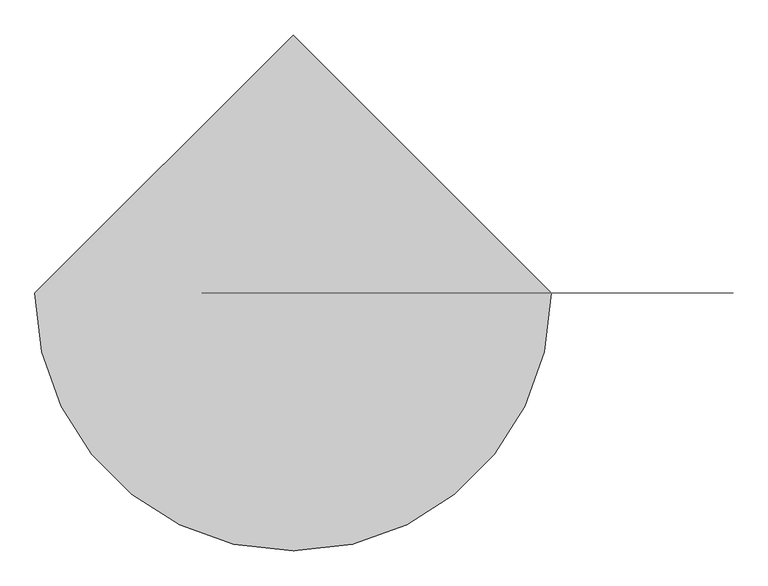
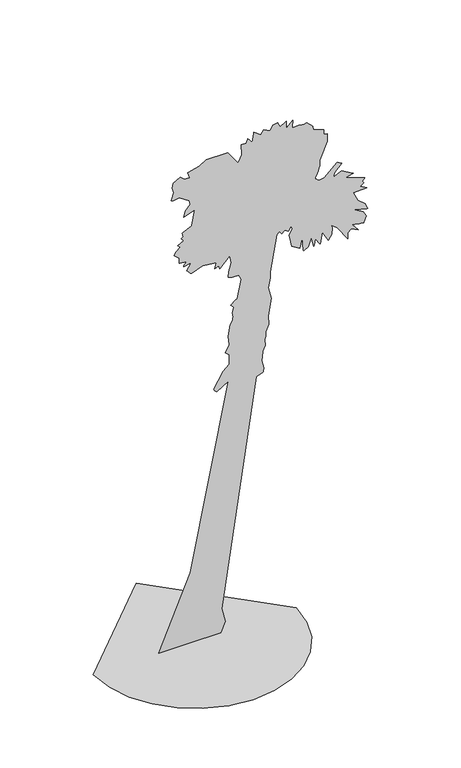
"""IFC4 building model written with IfcOpenShell, lengths in millimetres: proxy geometry, california fan palm 26448 : california fan palm 26448."""

import ifcopenshell
import ifcopenshell.guid

model = None  # the IFC model being written
_history = None  # IfcOwnerHistory: only IFC2X3 demands one
_inside = {}  # id of a spatial element -> (the spatial element, [elements in it])
_under = {}  # id of a project, library or spatial element -> (it, [spatial elements below it])
_declared = {}  # id of a project -> (the project, [libraries it declares])
_typed = {}  # id of a type object -> (the type object, [elements of that type])
_made_of = {}  # id of a material, layer set ... -> (it, [elements and type objects made of it])


def new_model(schema):
    """Start an empty IFC model of exactly this schema.

    Asked for "IFC4X3", IfcOpenShell would pick the latest addendum, in which some entities
    have other attributes; the version numbers below select the first issue.
    IFC2X3 requires an IfcOwnerHistory on every rooted entity: one is made here for all.
    """
    global model, _history
    if schema == "IFC4X3":
        model = ifcopenshell.file(schema_version=(4, 3, 0, 0))
    else:
        model = ifcopenshell.file(schema=schema)
    _inside.clear()
    _under.clear()
    _declared.clear()
    _typed.clear()
    _made_of.clear()
    _history = None
    if model.schema == "IFC2X3":
        org = make("IfcOrganization", Name="unknown")
        user = make(
            "IfcPersonAndOrganization",
            ThePerson=make("IfcPerson", FamilyName="unknown"),
            TheOrganization=org,
        )
        app = make(
            "IfcApplication",
            ApplicationDeveloper=org,
            Version="unknown",
            ApplicationFullName="unknown",
            ApplicationIdentifier="unknown",
        )
        _history = make(
            "IfcOwnerHistory",
            OwningUser=user,
            OwningApplication=app,
            ChangeAction="ADDED",
            CreationDate=0,
        )
    return model


def make(cls, **values):
    """One entity of the class cls with the attributes given. An attribute that is None is left unset."""
    return model.create_entity(
        cls, **{name: value for name, value in values.items() if value is not None}
    )


def rooted(cls, **values):
    """An entity with a GlobalId (a new one), such as an element, a storey or a relation."""
    return make(cls, GlobalId=ifcopenshell.guid.new(), OwnerHistory=_history, **values)


def si_unit(unit_type, name, prefix=None):
    """IfcSIUnit, for example si_unit("LENGTHUNIT", "METRE", prefix="MILLI")."""
    return make("IfcSIUnit", UnitType=unit_type, Prefix=prefix, Name=name)


def assignment(units):
    """IfcUnitAssignment: the units of a project."""
    return None if units is None else make("IfcUnitAssignment", Units=units)


def point(xyz):
    """IfcCartesianPoint."""
    return None if xyz is None else make("IfcCartesianPoint", Coordinates=xyz)


def direction(xyz):
    """IfcDirection."""
    return None if xyz is None else make("IfcDirection", DirectionRatios=xyz)


def frame(location, z_axis=None, x_axis=None):
    """IfcAxis2Placement3D, a coordinate frame: its origin and axes. An axis left out is left unset."""
    return make(
        "IfcAxis2Placement3D",
        Location=point(location),
        Axis=direction(z_axis),
        RefDirection=direction(x_axis),
    )


def origin():
    """The frame at (0, 0, 0) with its axes left unset."""
    return frame((0.0, 0.0, 0.0))


def place(relative_to, where):
    """IfcLocalPlacement: puts the frame where relative to a parent placement (None: the world)."""
    return make(
        "IfcLocalPlacement", PlacementRelTo=relative_to, RelativePlacement=where
    )


def context(
    kind, dimensions, precision=None, world=None, true_north=None, identifier=None
):
    """IfcGeometricRepresentationContext, for example the 3D "Model" context."""
    return make(
        "IfcGeometricRepresentationContext",
        ContextIdentifier=identifier,
        ContextType=kind,
        CoordinateSpaceDimension=dimensions,
        Precision=precision,
        WorldCoordinateSystem=world,
        TrueNorth=true_north,
    )


def project(units=None, contexts=None):
    """IfcProject with its units and contexts."""
    return rooted(
        "IfcProject",
        Name="project",
        RepresentationContexts=contexts,
        UnitsInContext=assignment(units),
    )


def spatial(cls, under=None, at=None, **own):
    """A site, building, storey or space (cls), placed at a placement, below another one or the project."""
    s = rooted(cls, ObjectPlacement=at, **own)
    if under is not None:
        _under.setdefault(under.id(), (under, []))[1].append(s)
    return s


def point_list(points):
    """IfcCartesianPointList2D or 3D."""
    cls = (
        "IfcCartesianPointList2D" if len(points[0]) == 2 else "IfcCartesianPointList3D"
    )
    return make(cls, CoordList=points)


def triangles(points, corners, closed=None, point_numbers=None):
    """IfcTriangulatedFaceSet: each triangle names its three corners, points numbered from 1."""
    return make(
        "IfcTriangulatedFaceSet",
        Coordinates=point_list(points),
        Closed=closed,
        CoordIndex=corners,
        PnIndex=point_numbers,
    )


def shape(context_of_items, identifier, shape_type, items):
    """IfcShapeRepresentation: the items that make up one representation, for example the "Body"."""
    return make(
        "IfcShapeRepresentation",
        ContextOfItems=context_of_items,
        RepresentationIdentifier=identifier,
        RepresentationType=shape_type,
        Items=items,
    )


def source(mapping_origin, context_of_items, identifier, shape_type, items):
    """IfcRepresentationMap: a shape defined once, which mapped items show again and again."""
    return make(
        "IfcRepresentationMap",
        MappingOrigin=mapping_origin,
        MappedRepresentation=shape(context_of_items, identifier, shape_type, items),
    )


def transform(
    local_origin,
    x_axis=None,
    y_axis=None,
    z_axis=None,
    scale=None,
    scale2=None,
    scale3=None,
    uniform=True,
):
    """IfcCartesianTransformationOperator3D, or its non-uniform kind. x_axis, y_axis, z_axis: its Axis1, 2, 3."""
    if uniform:
        return make(
            "IfcCartesianTransformationOperator3D",
            Axis1=direction(x_axis),
            Axis2=direction(y_axis),
            LocalOrigin=point(local_origin),
            Scale=scale,
            Axis3=direction(z_axis),
        )
    return make(
        "IfcCartesianTransformationOperator3DnonUniform",
        Axis1=direction(x_axis),
        Axis2=direction(y_axis),
        LocalOrigin=point(local_origin),
        Scale=scale,
        Axis3=direction(z_axis),
        Scale2=scale2,
        Scale3=scale3,
    )


def mapped(mapping_source, mapping_target):
    """IfcMappedItem: shows the shape of a source again, moved by a transform."""
    return make(
        "IfcMappedItem", MappingSource=mapping_source, MappingTarget=mapping_target
    )


def made_of(thing, what):
    """Note that an element or type object is made of a material, layer set ...; save() writes the relation."""
    if what is not None:
        _made_of.setdefault(what.id(), (what, []))[1].append(thing)
    return thing


def element(
    cls,
    number,
    at=None,
    inside=None,
    cuts=None,
    type_object=None,
    material=None,
    context=None,
    identifier="Body",
    shape_type=None,
    held_by="IfcProductDefinitionShape",
    body=None,
    shapes=None,
    **own,
):
    """One element of the class cls, such as IfcWall. Its Tag is "e" and its number.

    at: its placement. inside: the storey or other place that contains it. cuts: it is an
    opening in that element (IfcRelVoidsElement). A single representation is given by context,
    identifier, shape_type and body (its items); several are given by shapes. held_by: the class
    of the entity that holds the representations. save() writes the other relations.
    """
    e = rooted(cls, Tag="e%d" % number, ObjectPlacement=at, **own)
    if body is not None:
        shapes = [shape(context, identifier, shape_type, body)]
    if shapes is not None:
        e.Representation = make(held_by, Representations=shapes)
    if inside is not None:
        _inside.setdefault(inside.id(), (inside, []))[1].append(e)
    if cuts is not None:
        rooted(
            "IfcRelVoidsElement", RelatingBuildingElement=cuts, RelatedOpeningElement=e
        )
    if type_object is not None:
        _typed.setdefault(type_object.id(), (type_object, []))[1].append(e)
    return made_of(e, material)


def aggregate(whole, parts):
    """IfcRelAggregates: a whole, such as a stair, and the parts it consists of."""
    return rooted("IfcRelAggregates", RelatingObject=whole, RelatedObjects=parts)


def save(model, path):
    """Write the relations noted so far, then the file.

    IfcRelAggregates (storeys below a building ...), IfcRelContainedInSpatialStructure (elements
    in a storey), IfcRelDefinesByType, IfcRelAssociatesMaterial and IfcRelDeclares: one each for
    every whole, place, type object, material and project.
    """
    for whole, parts in _under.values():
        aggregate(whole, parts)
    for where, things in _inside.values():
        rooted(
            "IfcRelContainedInSpatialStructure",
            RelatedElements=things,
            RelatingStructure=where,
        )
    for kind, things in _typed.values():
        rooted("IfcRelDefinesByType", RelatedObjects=things, RelatingType=kind)
    for what, things in _made_of.values():
        rooted("IfcRelAssociatesMaterial", RelatedObjects=things, RelatingMaterial=what)
    for by, libraries in _declared.values():
        rooted("IfcRelDeclares", RelatingContext=by, RelatedDefinitions=libraries)
    model.write(path)


def entourage_5d10e8ee(model_context):
    return source(origin(), model_context, "Body", "Tessellation", [
        triangles([(-2230.6788128, 0.0, 0.0), (-2171.7626415, -511.0878808, 0.0), (-2003.8055969, -980.4489481, 0.0), (-1740.3231331, -1394.6991714, 0.0), (-1394.6991714, -1740.3231331, 0.0), (-980.4489481, -2003.8055969, 0.0), (-511.0878808, -2171.7626415, 0.0), (0.0, -2230.6788128, 0.0), (511.0878808, -2171.7626415, 0.0), (980.4489481, -2003.8055969, 0.0), (1394.6991714, -1740.3231331, 0.0), (1740.3231331, -1394.6991714, 0.0), (2003.8055969, -980.4489481, 0.0), (2171.7626415, -511.0878808, 0.0), (2230.6788128, 0.0, 0.0), (0.0, 2230.6788128, 0.0), (1664.2176041, 0.0, 11296.8139435), (1716.9665646, 0.0, 11409.2663818), (1822.5957275, 0.0, 11429.86745), (1831.5184387, 0.0, 11420.4191895), (1867.2094288, 0.0, 11334.210498), (1869.9649292, 0.0, 11312.4281067), (2015.4839539, 0.0, 11398.3751862), (2017.4521477, 0.0, 11231.8609314), (2029.3928432, 0.0, 11239.7348694), (2152.211364, 0.0, 11376.1997955), (2149.9806862, 0.0, 11207.8484436), (2152.473848, 0.0, 11197.3514099), (2288.0203709, 0.0, 11209.0297668), (2303.3726315, 0.0, 11206.5368958), (2322.5303284, 0.0, 11201.6813782), (2343.1312511, 0.0, 11196.0398621), (2362.6825287, 0.0, 11190.7901825), (2378.8220959, 0.0, 11187.6415375), (2392.5998886, 0.0, 11190.1344086), (2470.1486435, 0.0, 11209.9483154), (2596.1165359, 0.0, 11074.5333252), (2606.0888924, 0.0, 10999.6088287), (2622.0972176, 0.0, 10989.2420197), (2841.8846741, 0.0, 10912.2188141), (2834.4054794, 0.0, 10804.8835052), (2918.2526871, 0.0, 10792.4179871), (2914.3162994, 0.0, 10622.229538), (2746.3591095, 0.0, 10233.4358276), (2746.8840775, 0.0, 10223.5945679), (2748.4586906, 0.0, 10207.4548553), (2750.2957878, 0.0, 10187.6409485), (2752.0014977, 0.0, 10166.9096558), (2753.1825302, 0.0, 10147.8829102), (2752.5264656, 0.0, 10129.2503265), (2746.4904968, 0.0, 10101.3008698), (2732.5814621, 0.0, 10059.0487976), (2713.4239105, 0.0, 10006.1694672), (2692.2981651, 0.0, 9950.4019409), (2672.3531616, 0.0, 9899.7527069), (2657.000901, 0.0, 9861.830603), (2649.652803, 0.0, 9844.3793427), (2655.1638039, 0.0, 9835.7194061), (2666.9732574, 0.0, 9823.9096619), (2682.588002, 0.0, 9810.3942078), (2699.9087471, 0.0, 9796.4857544), (2716.8356209, 0.0, 9783.8888489), (2731.1382362, 0.0, 9773.7848145), (2743.9973351, 0.0, 9768.1421356), (2762.8924026, 0.0, 9771.5535553), (2783.4934708, 0.0, 9776.0149109), (2805.8002487, 0.0, 9781.0018158), (2826.6638008, 0.0, 9785.987558), (2846.6085136, 0.0, 9790.8430756), (3136.3344337, 0.0, 10050.2574738), (3236.3213539, 0.0, 9997.9025299), (3081.0921661, 0.0, 9835.4566315), (3047.3698059, 0.0, 9739.0125183), (3230.9414497, 0.0, 9821.1540161), (3471.198587, 0.0, 9683.1141861), (3486.2886543, 0.0, 9668.9429581), (3314.6575607, 0.0, 9631.5464035), (3745.0472786, 0.0, 9483.4031204), (3683.7693329, 0.0, 9424.0927872), (3714.4738541, 0.0, 9372.0000366), (3638.7619057, 0.0, 9318.7265442), (3786.6429955, 0.0, 9226.0874313), (3491.0122032, 0.0, 9221.3638824), (3589.5558975, 0.0, 9011.2860077), (3750.2957954, 0.0, 8872.4595978), (3802.1263527, 0.0, 8753.0523514), (3802.3888367, 0.0, 8743.6046722), (3785.8555435, 0.0, 8741.1118011), (3521.0609505, 0.0, 8817.3484268), (3708.9628532, 0.0, 8702.927504), (3773.3900253, 0.0, 8589.950679), (3773.3900253, 0.0, 8579.0594833), (3723.3965652, 0.0, 8451.5172684), (3722.7405006, 0.0, 8439.9702988), (3582.3388962, 0.0, 8467.3942062), (3469.6239738, 0.0, 8483.9274994), (3593.2298012, 0.0, 8317.5452133), (3446.0050667, 0.0, 8391.1575806), (3364.6510208, 0.0, 8326.0743439), (3364.9135048, 0.0, 8189.871611), (3139.2211761, 0.0, 8528.6724426), (3001.4438301, 0.0, 8636.6635254), (3024.9316406, 0.0, 8566.4625778), (3019.5517365, 0.0, 8420.4185852), (2940.4283684, 0.0, 8304.6861145), (2805.2752808, 0.0, 8540.6129929), (2760.1370476, 0.0, 8283.0351105), (2749.7708199, 0.0, 8292.6141769), (2653.9827713, 0.0, 8439.0517502), (2626.9524445, 0.0, 8297.7313065), (2620.9164757, 0.0, 8283.0351105), (2579.5832428, 0.0, 8449.8115585), (2567.9048859, 0.0, 8491.0131134), (2498.0978096, 0.0, 8313.2152451), (2400.9976318, 0.0, 8247.8692337), (2391.943824, 0.0, 8267.9453339), (2363.6010773, 0.0, 8580.3716125), (2316.2318756, 0.0, 8342.0826691), (2134.3659416, 0.0, 8446.7931381), (2079.2550613, 0.0, 8724.578508), (2142.2390076, 0.0, 8848.577916), (2140.5331524, 0.0, 8863.4054993), (2136.7278614, 0.0, 8876.1332108), (2131.7416832, 0.0, 8889.1236969), (2126.493021, 0.0, 8901.1956345), (2118.2263744, 0.0, 8911.5618622), (2064.821204, 0.0, 8836.1123978), (2061.278397, 0.0, 8825.74617), (1984.5168034, 0.0, 8874.5588882), (1971.6575592, 0.0, 8870.8846939), (1961.5539608, 0.0, 8863.4054993), (1929.4059231, 0.0, 8825.3525894), (1918.6462601, 0.0, 8820.3662659), (1866.2908802, 0.0, 8885.1873093), (1856.7121044, 0.0, 8882.4316635), (1845.5587154, 0.0, 8875.3460495), (1833.7492619, 0.0, 8865.5047897), (1822.2021469, 0.0, 8854.2200134), (1811.8360645, 0.0, 8842.9358185), (1800.8139175, 0.0, 8829.6825577), (1660.4123131, 0.0, 8018.3716141), (1661.7244423, 0.0, 7883.0874298), (1618.029435, 0.0, 7666.7116837), (1684.0312202, 0.0, 7392.9946701), (1613.6993214, 0.0, 6996.1962158), (1630.1013725, 0.0, 6826.0083481), (1628.2642754, 0.0, 6813.1492493), (1565.0179905, 0.0, 6658.9697067), (1565.0179905, 0.0, 6648.2098984), (1564.7555065, 0.0, 6634.432251), (1564.2306839, 0.0, 6619.0802811), (1564.0994419, 0.0, 6603.3341492), (1564.3619259, 0.0, 6588.6379532), (1566.3301197, 0.0, 6572.10466), (1566.0677811, 0.0, 6561.3448517), (1562.0000061, 0.0, 6547.1736237), (1555.9640373, 0.0, 6528.54104), (1549.2720039, 0.0, 6508.2021652), (1542.9736965, 0.0, 6489.176001), (1536.6752438, 0.0, 6470.41203), (1549.6657299, 0.0, 6358.8781403), (1547.8286327, 0.0, 6349.0368805), (1519.879612, 0.0, 6273.9809967), (1509.1198036, 0.0, 6246.9500885), (1500.7219151, 0.0, 6225.4310532), (1496.3918015, 0.0, 6213.6213089), (1479.0712017, 0.0, 6016.271727), (1517.6489342, 0.0, 5834.537471), (1516.3366596, 0.0, 5819.7098877), (1513.5811592, 0.0, 5801.6016907), (1510.1695942, 0.0, 5782.7069138), (1506.6266418, 0.0, 5765.255072), (1502.4277702, 0.0, 5747.9346176), (1492.9802364, 0.0, 5740.5862289), (1349.2983089, 0.0, 5680.8828964), (595.4600201, 0.0, 547.8284798), (673.9273962, 0.0, 229.1038392), (568.9542978, 0.0, 0.0), (-790.1851255, 0.0, 0.0), (-95.6567521, 0.0, 1632.0695663), (739.9292542, 0.0, 5779.1641068), (737.436165, 0.0, 5791.104657), (723.0023804, 0.0, 5788.3490112), (497.4413664, 0.0, 5642.1742126), (481.6954162, 0.0, 5644.929277), (467.1303895, 0.0, 5652.2776657), (442.9865507, 0.0, 5676.2901535), (421.4670794, 0.0, 5718.8044189), (623.2778715, 0.0, 6073.2199951), (759.0868784, 0.0, 6187.6403366), (764.0731293, 0.0, 6248.393605), (761.5799675, 0.0, 6329.354361), (759.4805317, 0.0, 6365.176593), (758.0371605, 0.0, 6391.1569839), (755.0191761, 0.0, 6405.9845673), (666.1856449, 0.0, 6482.8775482), (763.548234, 0.0, 6634.301445), (735.9927938, 0.0, 6838.6052536), (766.6974604, 0.0, 7041.3347397), (776.8010588, 0.0, 7092.5089417), (840.0474163, 0.0, 7190.1337967), (839.522521, 0.0, 7202.4679276), (839.653763, 0.0, 7214.1462845), (840.3098276, 0.0, 7226.8745773), (841.2283762, 0.0, 7239.2087082), (843.0654007, 0.0, 7253.5113235), (843.459054, 0.0, 7264.4025192), (841.4907875, 0.0, 7278.1801666), (838.3415611, 0.0, 7296.025589), (834.5362701, 0.0, 7315.1831406), (830.9934631, 0.0, 7332.8971756), (827.1881721, 0.0, 7349.5618561), (858.9425566, 0.0, 7476.4482971), (792.0222227, 0.0, 7542.3186951), (801.9946518, 0.0, 7559.2455688), (893.5836834, 0.0, 7626.0345154), (936.6226988, 0.0, 7645.4548416), (1020.8635597, 0.0, 8067.9714935), (970.6076883, 0.0, 8186.4601913), (830.0749146, 0.0, 8178.4560287), (740.9790447, 0.0, 8214.1468735), (747.8022474, 0.0, 8345.4940887), (801.8634098, 0.0, 8532.8710236), (775.3576876, 0.0, 8707.5202469), (545.597802, 0.0, 8480.6468857), (527.0962787, 0.0, 8557.4084793), (442.0680385, 0.0, 8522.5053772), (472.772705, 0.0, 8646.6361725), (175.6987596, 0.0, 8679.0464035), (149.3242611, 0.0, 8677.3406937), (-68.4949607, 0.0, 8593.099324), (-83.7160656, 0.0, 8594.6742279), (-100.2493315, 0.0, 8606.0898102), (-163.6268583, 0.0, 8679.0464035), (-174.6490235, 0.0, 8687.0505661), (-73.2187503, 0.0, 8837.8181076), (-247.211691, 0.0, 8810.3942001), (-243.8000715, 0.0, 8822.3347504), (-191.1822985, 0.0, 8889.9108582), (-182.5220168, 0.0, 8896.9970535), (-226.4795081, 0.0, 8901.4584091), (-326.8600634, 0.0, 8910.7747009), (-336.4388391, 0.0, 8914.1861206), (-338.5383113, 0.0, 9032.0184631), (-454.139976, 0.0, 9130.9554474), (-421.729527, 0.0, 9200.631427), (-316.4939446, 0.0, 9287.7592484), (-374.0979504, 0.0, 9343.1326126), (-245.112237, 0.0, 9404.9352356), (-247.8677738, 0.0, 9414.1207214), (-255.0846843, 0.0, 9424.7491425), (-300.8792001, 0.0, 9470.2812469), (-254.166172, 0.0, 9507.1528336), (-275.2920083, 0.0, 9598.0862366), (-268.468751, 0.0, 9606.3525925), (-79.1234862, 0.0, 9686.3947998), (-65.8706341, 0.0, 9707.3894485), (-0.1312164, 0.0, 10040.1546021), (-244.7185837, 0.0, 9956.7003937), (-207.9780029, 0.0, 10078.3383179), (-100.1181167, 0.0, 10203.780661), (-126.0989619, 0.0, 10300.0933868), (-346.8049579, 0.0, 10440.889444), (-468.442555, 0.0, 10419.7628265), (-522.8973707, 0.0, 10436.8210876), (-465.9494296, 0.0, 10603.5969543), (-492.9800108, 0.0, 10720.6421356), (-468.8362083, 0.0, 10823.2533142), (-318.9870701, 0.0, 10910.9061035), (-233.6964004, 0.0, 10839.2616394), (-108.1223157, 0.0, 10825.353186), (-151.5549389, 0.0, 10960.7681763), (96.9689176, 0.0, 11018.8971863), (255.6095432, 0.0, 11124.9197845), (725.2330582, 0.0, 11114.0285889), (954.2056372, 0.0, 10789.530954), (960.8976706, 0.0, 10798.7164398), (1037.2656109, 0.0, 10964.7051453), (1025.8498106, 0.0, 11198.2699585), (1137.9085957, 0.0, 11192.758667), (1136.4652245, 0.0, 11204.0440247), (1141.5826447, 0.0, 11231.8609314), (1162.0524708, 0.0, 11273.5886169), (1170.1878754, 0.0, 11283.6914886), (1265.188472, 0.0, 11172.5517609), (1295.1058319, 0.0, 11376.1997955), (1299.9609135, 0.0, 11390.6337982), (1447.8417126, 0.0, 11287.365683), (1520.9292572, 0.0, 11379.6112152)], [[15, 16, 1], [14, 15, 1], [14, 1, 2], [13, 14, 2], [13, 2, 3], [13, 3, 4], [12, 13, 4], [11, 12, 4], [11, 4, 5], [11, 5, 6], [11, 6, 7], [11, 7, 8], [11, 8, 9], [11, 9, 10], [266, 267, 268], [266, 268, 269], [266, 269, 270], [271, 272, 273], [278, 279, 280], [283, 284, 285], [282, 283, 285], [281, 282, 285], [280, 281, 285], [278, 280, 285], [277, 278, 285], [286, 287, 288], [285, 286, 288], [277, 285, 288], [288, 289, 17], [277, 288, 17], [276, 277, 17], [18, 19, 20], [17, 18, 20], [17, 20, 21], [17, 21, 22], [22, 23, 24], [25, 26, 27], [25, 27, 28], [24, 25, 28], [35, 36, 37], [35, 37, 38], [34, 35, 38], [39, 40, 41], [41, 42, 43], [41, 43, 44], [39, 41, 44], [38, 39, 44], [34, 38, 44], [33, 34, 44], [32, 33, 44], [31, 32, 44], [30, 31, 44], [29, 30, 44], [28, 29, 44], [24, 28, 44], [70, 71, 72], [69, 70, 72], [69, 72, 73], [75, 76, 77], [74, 75, 77], [73, 74, 77], [77, 78, 79], [79, 80, 81], [77, 79, 81], [81, 82, 83], [77, 81, 83], [73, 77, 83], [86, 87, 88], [85, 86, 88], [84, 85, 88], [84, 88, 89], [83, 84, 89], [93, 94, 95], [92, 93, 95], [91, 92, 95], [90, 91, 95], [90, 95, 96], [96, 97, 98], [99, 100, 101], [98, 99, 101], [96, 98, 101], [90, 96, 101], [89, 90, 101], [89, 101, 102], [83, 89, 102], [73, 83, 102], [69, 73, 102], [68, 69, 102], [67, 68, 102], [66, 67, 102], [65, 66, 102], [64, 65, 102], [104, 105, 106], [103, 104, 106], [102, 103, 106], [64, 102, 106], [106, 107, 108], [106, 108, 109], [110, 111, 112], [109, 110, 112], [106, 109, 112], [106, 112, 113], [64, 106, 113], [114, 115, 116], [113, 114, 116], [113, 116, 117], [64, 113, 117], [117, 118, 119], [117, 119, 120], [117, 120, 121], [64, 117, 121], [64, 121, 122], [64, 122, 123], [64, 123, 124], [64, 124, 125], [64, 125, 126], [63, 64, 126], [62, 63, 126], [61, 62, 126], [60, 61, 126], [59, 60, 126], [58, 59, 126], [57, 58, 126], [127, 128, 129], [126, 127, 129], [57, 126, 129], [57, 129, 130], [131, 132, 133], [131, 133, 134], [130, 131, 134], [57, 130, 134], [177, 178, 179], [176, 177, 179], [176, 179, 180], [175, 176, 180], [175, 180, 181], [175, 181, 182], [187, 188, 189], [186, 187, 189], [185, 186, 189], [184, 185, 189], [183, 184, 189], [182, 183, 189], [182, 189, 190], [175, 182, 190], [175, 190, 191], [174, 175, 191], [173, 174, 191], [172, 173, 191], [171, 172, 191], [170, 171, 191], [169, 170, 191], [168, 169, 191], [167, 168, 191], [166, 167, 191], [166, 191, 192], [165, 166, 192], [165, 192, 193], [164, 165, 193], [164, 193, 194], [163, 164, 194], [163, 194, 195], [162, 163, 195], [161, 162, 195], [160, 161, 195], [159, 160, 195], [158, 159, 195], [157, 158, 195], [156, 157, 195], [155, 156, 195], [154, 155, 195], [153, 154, 195], [152, 153, 195], [151, 152, 195], [150, 151, 195], [149, 150, 195], [148, 149, 195], [148, 195, 196], [148, 196, 197], [148, 197, 198], [148, 198, 199], [147, 148, 199], [146, 147, 199], [145, 146, 199], [145, 199, 200], [145, 200, 201], [144, 145, 201], [144, 201, 202], [144, 202, 203], [144, 203, 204], [144, 204, 205], [144, 205, 206], [144, 206, 207], [143, 144, 207], [143, 207, 208], [143, 208, 209], [143, 209, 210], [143, 210, 211], [143, 211, 212], [143, 212, 213], [213, 214, 215], [213, 215, 216], [213, 216, 217], [143, 213, 217], [143, 217, 218], [142, 143, 218], [141, 142, 218], [141, 218, 219], [220, 221, 222], [220, 222, 223], [219, 220, 223], [141, 219, 223], [140, 141, 223], [140, 223, 224], [139, 140, 224], [138, 139, 224], [224, 225, 226], [226, 227, 228], [224, 226, 228], [234, 235, 236], [233, 234, 236], [232, 233, 236], [231, 232, 236], [230, 231, 236], [229, 230, 236], [236, 237, 238], [236, 238, 239], [236, 239, 240], [242, 243, 244], [241, 242, 244], [244, 245, 246], [244, 246, 247], [241, 244, 247], [240, 241, 247], [247, 248, 249], [240, 247, 249], [236, 240, 249], [229, 236, 249], [228, 229, 249], [224, 228, 249], [138, 224, 249], [137, 138, 249], [137, 249, 250], [136, 137, 250], [135, 136, 250], [135, 250, 251], [251, 252, 253], [135, 251, 253], [253, 254, 255], [253, 255, 256], [135, 253, 256], [135, 256, 257], [135, 257, 258], [134, 135, 258], [57, 134, 258], [56, 57, 258], [55, 56, 258], [54, 55, 258], [53, 54, 258], [52, 53, 258], [51, 52, 258], [50, 51, 258], [49, 50, 258], [48, 49, 258], [47, 48, 258], [46, 47, 258], [45, 46, 258], [44, 45, 258], [24, 44, 258], [22, 24, 258], [17, 22, 258], [276, 17, 258], [259, 260, 261], [258, 259, 261], [276, 258, 261], [276, 261, 262], [275, 276, 262], [274, 275, 262], [273, 274, 262], [271, 273, 262], [271, 262, 263], [270, 271, 263], [266, 270, 263], [266, 263, 264], [266, 264, 265]], closed=False),
    ])


if __name__ == "__main__":
    model = new_model("IFC4")
    model_context = context("Model", 3, world=origin())
    ifc_project = project(units=[si_unit("LENGTHUNIT", "METRE", prefix="MILLI")], contexts=[model_context])
    site = spatial("IfcSite", under=ifc_project)
    building = spatial("IfcBuilding", under=site)
    placement = place(None, origin())
    entourage_shape = entourage_5d10e8ee(model_context)
    element("IfcBuildingElementProxy", 1, Name="california fan palm 26448 : california fan palm 26448", ObjectType="california fan palm 26448 : california fan palm 26448", at=placement, inside=building, context=model_context, shape_type="MappedRepresentation", body=[
        mapped(entourage_shape, transform((0.0, 0.0, 0.0), x_axis=(1.0, 0.0, 0.0), y_axis=(0.0, 1.0, 0.0), z_axis=(0.0, 0.0, 1.0))),
    ])
    save(model, "model.ifc")

# Revit data of these elements
# Type "california fan palm 26448 : california fan palm 26448"
#   built-in parameter 1005195 = "RPC-16-1C97-WEA8-8LP7-XB2E-SRLV-LDXM-F4"
#   Height = 0
